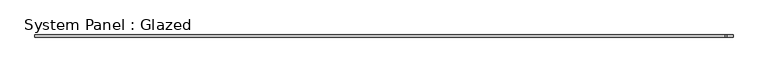
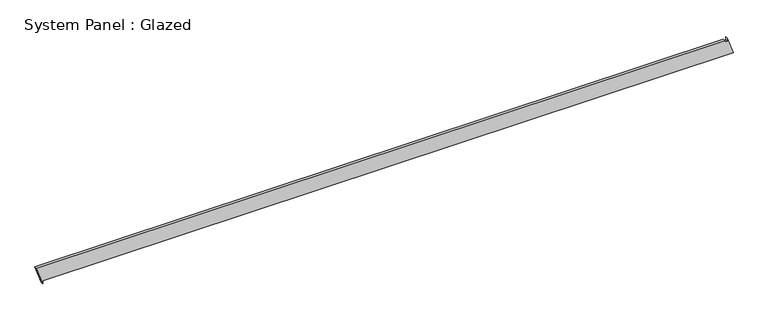
"""IFC4 building model written with IfcOpenShell, lengths in millimetres: plate geometry, System Panel : Glazed."""

from ifc_helpers import new_model, si_unit, frame, origin, place, context, project, spatial, polyline, outline, extrude, source, transform, mapped, element, save


def system_panel_glazed_255fc0b9(model_context):
    return source(origin(), model_context, "Body", "SweptSolid", [
        extrude(outline(polyline([(0.0, -3956.1046567), (35.3553391, -3956.1046567), (35.3553391, 4031.0223473), (235.5290854, 3961.7982225), (200.1737464, 3961.7984265), (200.1735967, 3935.8556462), (216.0829691, 3932.4976189), (216.0408196, -4031.0223473), (0.0, -3956.1046567)])), frame((0.0, -49.5, 0.0), z_axis=(0.0, 1.0, 0.0), x_axis=(0.0, 0.0, 1.0)), (0.0, 0.0, 1.0), 25.0),
    ])


if __name__ == "__main__":
    model = new_model("IFC4")
    model_context = context("Model", 3, world=origin())
    ifc_project = project(units=[si_unit("LENGTHUNIT", "METRE", prefix="MILLI")], contexts=[model_context])
    site = spatial("IfcSite", under=ifc_project)
    building = spatial("IfcBuilding", under=site)
    placement = place(None, origin())
    system_panel_glazed_shape = system_panel_glazed_255fc0b9(model_context)
    element("IfcPlate", 1, ObjectType="System Panel : Glazed", at=placement, inside=building, context=model_context, shape_type="MappedRepresentation", body=[
        mapped(system_panel_glazed_shape, transform((0.0, 0.0, 0.0), x_axis=(1.0, 0.0, 0.0), y_axis=(0.0, 1.0, 0.0), z_axis=(0.0, 0.0, 1.0))),
    ])
    save(model, "model.ifc")

# Revit data of these elements
# Element 1 (IfcPlate, "System Panel : Glazed")
#   Materials on its faces: "Glass"
# Materials
#   "Glass": class "Glass", colour RGB 218 227 224, transparency 0.85, Description = "Soda Lime Glass", Cost = 0
